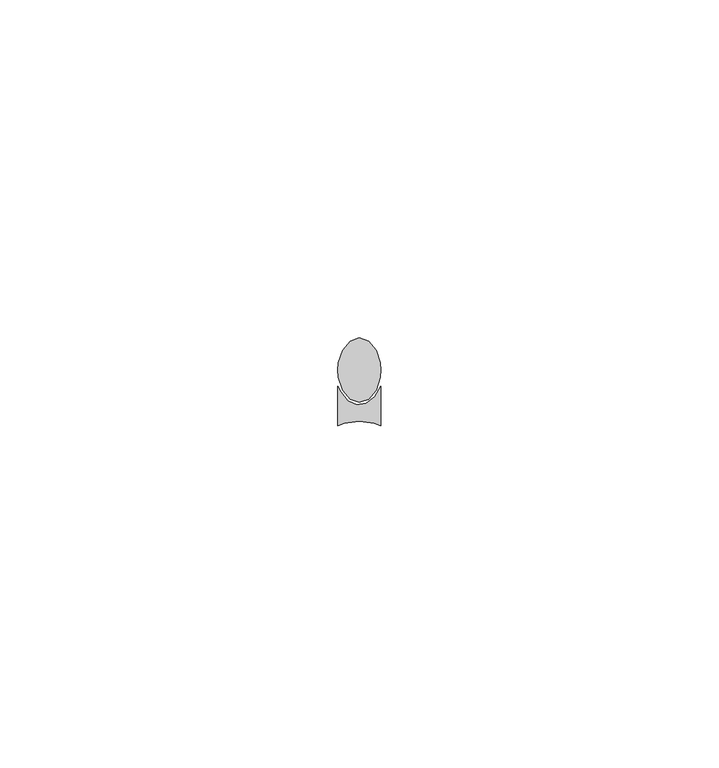
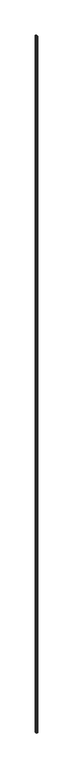
"""IFC4 building model written with IfcOpenShell, lengths in millimetres: proxy geometry, Generic Models 11:Generic Models 1:306267:Generic Models 1:306267 : Generic Models 11:Generic Models 1:306267:300405:Generic Models 1:306267:Generic Models 1:306267 : Generic Models 11:Generic Models 1:306267:300405 : Generic Models 11:Generic Models 1:306267:Generic Models 1:306267 : Generic Models 11:Generic Models 1:306267:300405:11 : Generic Models 11:Generic Models 1:306267:Generic Models 1:306267 : Generic Models 11:Generic Models 1:306267:300405:Generic Models 1:306267:Generic Models 1:306267 : Generic Models 11:Generic Models 1:306267:300405 : Generic Models 11:Generic Models 1:306267:Generic Models 1:306267 : Generic Models 11:Generic Models 1:306267:300405:300182."""

from ifc_helpers import new_model, si_unit, origin, origin_with_axes, place, context, project, spatial, polyline, outline, extrude, source, transform, mapped, element, save


def generic_models_3330a79a(model_context):
    return source(origin(), model_context, "Body", "SweptSolid", [
        extrude(outline(polyline([(592757.2216431, -579082.4586403), (592756.116909, -579081.1371463), (592755.5038278, -579079.2275321), (592755.4242239, -579078.1677761), (592755.5038278, -579077.1080202), (592756.116909, -579075.1984059), (592757.2216431, -579073.8769119), (592758.5992239, -579073.4052761), (592759.9768048, -579073.8769119), (592761.0815389, -579075.1984059), (592761.6946201, -579077.1080202), (592761.7742239, -579078.1677761), (592761.6946201, -579079.2275321), (592761.0815389, -579081.1371463), (592759.9768048, -579082.4586403), (592758.5992239, -579082.9302761), (592757.2216431, -579082.4586403)])), origin_with_axes(), (0.0, 0.0, 1.0), 3695.7),
        extrude(outline(polyline([(592760.8084607, -579086.0220872), (592758.5992239, -579085.7084011), (592756.3899872, -579086.0220872), (592755.4242239, -579086.3994958), (592755.4242239, -579080.5314037), (592755.8105415, -579081.3916847), (592756.894027, -579082.7012598), (592758.2442747, -579083.3016133), (592759.650051, -579083.0988254), (592760.8914351, -579082.1246204), (592761.7742239, -579080.5314037), (592761.7742239, -579086.3994958), (592760.8084607, -579086.0220872)])), origin_with_axes(), (0.0, 0.0, 1.0), 3695.7),
    ])


if __name__ == "__main__":
    model = new_model("IFC4")
    model_context = context("Model", 3, world=origin())
    ifc_project = project(units=[si_unit("LENGTHUNIT", "METRE", prefix="MILLI")], contexts=[model_context])
    site = spatial("IfcSite", under=ifc_project)
    building = spatial("IfcBuilding", under=site)
    placement = place(None, origin())
    generic_models_shape = generic_models_3330a79a(model_context)
    element("IfcBuildingElementProxy", 1, Name="Generic Models 11:Generic Models 1:306267:Generic Models 1:306267 : Generic Models 11:Generic Models 1:306267:300405:Generic Models 1:306267:Generic Models 1:306267 : Generic Models 11:Generic Models 1:306267:300405 : Generic Models 11:Generic Models 1:306267:Generic Models 1:306267 : Generic Models 11:Generic Models 1:306267:300405:11 : Generic Models 11:Generic Models 1:306267:Generic Models 1:306267 : Generic Models 11:Generic Models 1:306267:300405:Generic Models 1:306267:Generic Models 1:306267 : Generic Models 11:Generic Models 1:306267:300405 : Generic Models 11:Generic Models 1:306267:Generic Models 1:306267 : Generic Models 11:Generic Models 1:306267:300405:300182", ObjectType="Generic Models 11:Generic Models 1:306267:Generic Models 1:306267 : Generic Models 11:Generic Models 1:306267:300405:Generic Models 1:306267:Generic Models 1:306267 : Generic Models 11:Generic Models 1:306267:300405 : Generic Models 11:Generic Models 1:306267:Generic Models 1:306267 : Generic Models 11:Generic Models 1:306267:300405:11 : Generic Models 11:Generic Models 1:306267:Generic Models 1:306267 : Generic Models 11:Generic Models 1:306267:300405:Generic Models 1:306267:Generic Models 1:306267 : Generic Models 11:Generic Models 1:306267:300405 : Generic Models 11:Generic Models 1:306267:Generic Models 1:306267 : Generic Models 11:Generic Models 1:306267:300405:300182", at=placement, inside=building, context=model_context, shape_type="MappedRepresentation", body=[
        mapped(generic_models_shape, transform((0.0, 0.0, 0.0), x_axis=(1.0, 0.0, 0.0), y_axis=(0.0, 1.0, 0.0), z_axis=(0.0, 0.0, 1.0))),
    ])
    save(model, "model.ifc")

# Revit data of these elements
# Type "Generic Models 11:Generic Models 1:306267:Generic Models 1:306267 : Generic Models 11:Generic Models 1:306267:300405:Generic Models 1:306267:Generic Models 1:306267 : Generic Models 11:Generic Models 1:306267:300405 : Generic Models 11:Generic Models 1:306267:Generic Models 1:306267 : Generic Models 11:Generic Models 1:306267:300405:11 : Generic Models 11:Generic Models 1:306267:Generic Models 1:306267 : Generic Models 11:Generic Models 1:306267:300405:Generic Models 1:306267:Generic Models 1:306267 : Generic Models 11:Generic Models 1:306267:300405 : Generic Models 11:Generic Models 1:306267:Generic Models 1:306267 : Generic Models 11:Generic Models 1:306267:300405:300182"
#   NameOverride = "Generic Models 11:Generic Models 1:306267:Generic Models 1:306267 : Generic Models 11:Generic Models 1:306267:300405:Generic Models 1:306267:Generic Models 1:306267 : Generic Models 11:Generic Models 1:306267:300405 : Generic Models 11:Generic Models 1:306267:Generic Models 1:306267 : Generic Models 11:Generic Models 1:306267:300405:300182"
#   ObjectTypeOverride = "Generic Models 1:306267:Generic Models 1:306267 : Generic Models 11:Generic Models 1:306267:300405 : Generic Models 11:Generic Models 1:306267:Generic Models 1:306267 : Generic Models 11:Generic Models 1:306267:300405"
#   Reference = "Generic Models 1"
#   Tag = "300182"
# Element 1 (IfcBuildingElementProxy, "Generic Models 11:Generic Models 1:306267:Generic Models 1:306267 : Generic Models 11:Generic Models 1:306267:300405:Generic Models 1:306267:Generic Models 1:306267 : Generic Models 11:Generic Models 1:306267:300405 : Generic Models 11:Generic Models 1:306267:Generic Models 1:306267 : Generic Models 11:Generic Models 1:306267:300405:11 : Generic Models 11:Generic Models 1:306267:Generic Models 1:306267 : Generic Models 11:Generic Models 1:306267:300405:Generic Models 1:306267:Generic Models 1:306267 : Generic Models 11:Generic Models 1:306267:300405 : Generic Models 11:Generic Models 1:306267:Generic Models 1:306267 : Generic Models 11:Generic Models 1:306267:300405:300182")
#   Materials on its faces: "SEALANT & BACKER ROD"
# Materials
#   "SEALANT & BACKER ROD": class "Unassigned", colour RGB 120 120 120, transparency 0, Cost = 0
